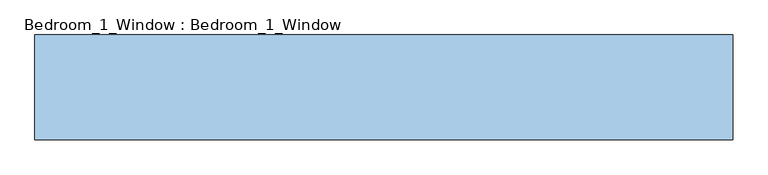
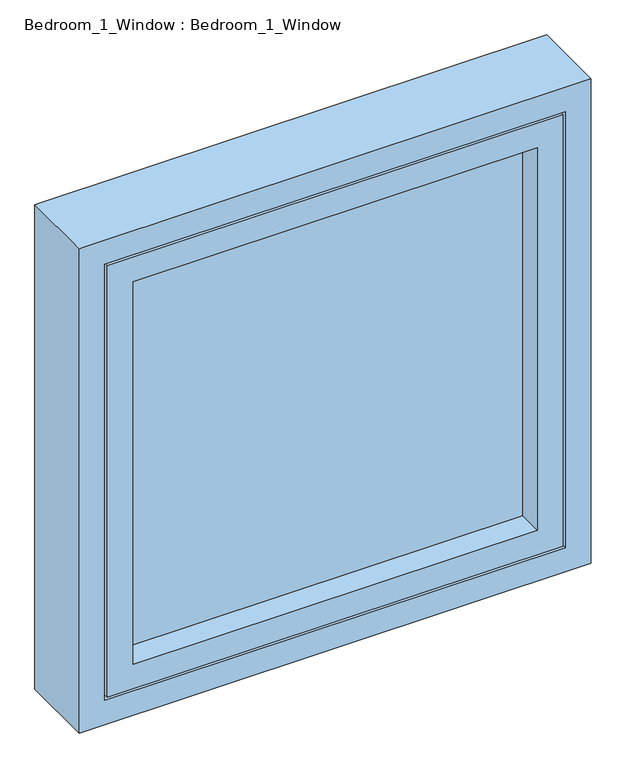
"""IFC4 building model written with IfcOpenShell, lengths in millimetres: window geometry, Bedroom_1_Window : Bedroom_1_Window."""

import ifcopenshell
import ifcopenshell.guid

model = None  # the IFC model being written
_history = None  # IfcOwnerHistory: only IFC2X3 demands one
_inside = {}  # id of a spatial element -> (the spatial element, [elements in it])
_under = {}  # id of a project, library or spatial element -> (it, [spatial elements below it])
_declared = {}  # id of a project -> (the project, [libraries it declares])
_typed = {}  # id of a type object -> (the type object, [elements of that type])
_made_of = {}  # id of a material, layer set ... -> (it, [elements and type objects made of it])


def new_model(schema):
    """Start an empty IFC model of exactly this schema.

    Asked for "IFC4X3", IfcOpenShell would pick the latest addendum, in which some entities
    have other attributes; the version numbers below select the first issue.
    IFC2X3 requires an IfcOwnerHistory on every rooted entity: one is made here for all.
    """
    global model, _history
    if schema == "IFC4X3":
        model = ifcopenshell.file(schema_version=(4, 3, 0, 0))
    else:
        model = ifcopenshell.file(schema=schema)
    _inside.clear()
    _under.clear()
    _declared.clear()
    _typed.clear()
    _made_of.clear()
    _history = None
    if model.schema == "IFC2X3":
        org = make("IfcOrganization", Name="unknown")
        user = make(
            "IfcPersonAndOrganization",
            ThePerson=make("IfcPerson", FamilyName="unknown"),
            TheOrganization=org,
        )
        app = make(
            "IfcApplication",
            ApplicationDeveloper=org,
            Version="unknown",
            ApplicationFullName="unknown",
            ApplicationIdentifier="unknown",
        )
        _history = make(
            "IfcOwnerHistory",
            OwningUser=user,
            OwningApplication=app,
            ChangeAction="ADDED",
            CreationDate=0,
        )
    return model


def make(cls, **values):
    """One entity of the class cls with the attributes given. An attribute that is None is left unset."""
    return model.create_entity(
        cls, **{name: value for name, value in values.items() if value is not None}
    )


def rooted(cls, **values):
    """An entity with a GlobalId (a new one), such as an element, a storey or a relation."""
    return make(cls, GlobalId=ifcopenshell.guid.new(), OwnerHistory=_history, **values)


def si_unit(unit_type, name, prefix=None):
    """IfcSIUnit, for example si_unit("LENGTHUNIT", "METRE", prefix="MILLI")."""
    return make("IfcSIUnit", UnitType=unit_type, Prefix=prefix, Name=name)


def assignment(units):
    """IfcUnitAssignment: the units of a project."""
    return None if units is None else make("IfcUnitAssignment", Units=units)


def point(xyz):
    """IfcCartesianPoint."""
    return None if xyz is None else make("IfcCartesianPoint", Coordinates=xyz)


def direction(xyz):
    """IfcDirection."""
    return None if xyz is None else make("IfcDirection", DirectionRatios=xyz)


def frame(location, z_axis=None, x_axis=None):
    """IfcAxis2Placement3D, a coordinate frame: its origin and axes. An axis left out is left unset."""
    return make(
        "IfcAxis2Placement3D",
        Location=point(location),
        Axis=direction(z_axis),
        RefDirection=direction(x_axis),
    )


def origin():
    """The frame at (0, 0, 0) with its axes left unset."""
    return frame((0.0, 0.0, 0.0))


def place(relative_to, where):
    """IfcLocalPlacement: puts the frame where relative to a parent placement (None: the world)."""
    return make(
        "IfcLocalPlacement", PlacementRelTo=relative_to, RelativePlacement=where
    )


def context(
    kind, dimensions, precision=None, world=None, true_north=None, identifier=None
):
    """IfcGeometricRepresentationContext, for example the 3D "Model" context."""
    return make(
        "IfcGeometricRepresentationContext",
        ContextIdentifier=identifier,
        ContextType=kind,
        CoordinateSpaceDimension=dimensions,
        Precision=precision,
        WorldCoordinateSystem=world,
        TrueNorth=true_north,
    )


def project(units=None, contexts=None):
    """IfcProject with its units and contexts."""
    return rooted(
        "IfcProject",
        Name="project",
        RepresentationContexts=contexts,
        UnitsInContext=assignment(units),
    )


def spatial(cls, under=None, at=None, **own):
    """A site, building, storey or space (cls), placed at a placement, below another one or the project."""
    s = rooted(cls, ObjectPlacement=at, **own)
    if under is not None:
        _under.setdefault(under.id(), (under, []))[1].append(s)
    return s


def polyline(points):
    """IfcPolyline through the points."""
    return make("IfcPolyline", Points=[point(p) for p in points])


def outline(outer, holes=None, kind="AREA"):
    """IfcArbitraryClosedProfileDef: a profile drawn as a closed curve; with holes, ...WithVoids."""
    if holes is None:
        return make("IfcArbitraryClosedProfileDef", ProfileType=kind, OuterCurve=outer)
    return make(
        "IfcArbitraryProfileDefWithVoids",
        ProfileType=kind,
        OuterCurve=outer,
        InnerCurves=holes,
    )


def extrude(swept, where, along, depth):
    """IfcExtrudedAreaSolid: the profile swept, set in the frame where, extruded along a direction by depth."""
    return make(
        "IfcExtrudedAreaSolid",
        SweptArea=swept,
        Position=where,
        ExtrudedDirection=direction(along),
        Depth=depth,
    )


def shape(context_of_items, identifier, shape_type, items):
    """IfcShapeRepresentation: the items that make up one representation, for example the "Body"."""
    return make(
        "IfcShapeRepresentation",
        ContextOfItems=context_of_items,
        RepresentationIdentifier=identifier,
        RepresentationType=shape_type,
        Items=items,
    )


def source(mapping_origin, context_of_items, identifier, shape_type, items):
    """IfcRepresentationMap: a shape defined once, which mapped items show again and again."""
    return make(
        "IfcRepresentationMap",
        MappingOrigin=mapping_origin,
        MappedRepresentation=shape(context_of_items, identifier, shape_type, items),
    )


def transform(
    local_origin,
    x_axis=None,
    y_axis=None,
    z_axis=None,
    scale=None,
    scale2=None,
    scale3=None,
    uniform=True,
):
    """IfcCartesianTransformationOperator3D, or its non-uniform kind. x_axis, y_axis, z_axis: its Axis1, 2, 3."""
    if uniform:
        return make(
            "IfcCartesianTransformationOperator3D",
            Axis1=direction(x_axis),
            Axis2=direction(y_axis),
            LocalOrigin=point(local_origin),
            Scale=scale,
            Axis3=direction(z_axis),
        )
    return make(
        "IfcCartesianTransformationOperator3DnonUniform",
        Axis1=direction(x_axis),
        Axis2=direction(y_axis),
        LocalOrigin=point(local_origin),
        Scale=scale,
        Axis3=direction(z_axis),
        Scale2=scale2,
        Scale3=scale3,
    )


def mapped(mapping_source, mapping_target):
    """IfcMappedItem: shows the shape of a source again, moved by a transform."""
    return make(
        "IfcMappedItem", MappingSource=mapping_source, MappingTarget=mapping_target
    )


def made_of(thing, what):
    """Note that an element or type object is made of a material, layer set ...; save() writes the relation."""
    if what is not None:
        _made_of.setdefault(what.id(), (what, []))[1].append(thing)
    return thing


def element(
    cls,
    number,
    at=None,
    inside=None,
    cuts=None,
    type_object=None,
    material=None,
    context=None,
    identifier="Body",
    shape_type=None,
    held_by="IfcProductDefinitionShape",
    body=None,
    shapes=None,
    **own,
):
    """One element of the class cls, such as IfcWall. Its Tag is "e" and its number.

    at: its placement. inside: the storey or other place that contains it. cuts: it is an
    opening in that element (IfcRelVoidsElement). A single representation is given by context,
    identifier, shape_type and body (its items); several are given by shapes. held_by: the class
    of the entity that holds the representations. save() writes the other relations.
    """
    e = rooted(cls, Tag="e%d" % number, ObjectPlacement=at, **own)
    if body is not None:
        shapes = [shape(context, identifier, shape_type, body)]
    if shapes is not None:
        e.Representation = make(held_by, Representations=shapes)
    if inside is not None:
        _inside.setdefault(inside.id(), (inside, []))[1].append(e)
    if cuts is not None:
        rooted(
            "IfcRelVoidsElement", RelatingBuildingElement=cuts, RelatedOpeningElement=e
        )
    if type_object is not None:
        _typed.setdefault(type_object.id(), (type_object, []))[1].append(e)
    return made_of(e, material)


def aggregate(whole, parts):
    """IfcRelAggregates: a whole, such as a stair, and the parts it consists of."""
    return rooted("IfcRelAggregates", RelatingObject=whole, RelatedObjects=parts)


def save(model, path):
    """Write the relations noted so far, then the file.

    IfcRelAggregates (storeys below a building ...), IfcRelContainedInSpatialStructure (elements
    in a storey), IfcRelDefinesByType, IfcRelAssociatesMaterial and IfcRelDeclares: one each for
    every whole, place, type object, material and project.
    """
    for whole, parts in _under.values():
        aggregate(whole, parts)
    for where, things in _inside.values():
        rooted(
            "IfcRelContainedInSpatialStructure",
            RelatedElements=things,
            RelatingStructure=where,
        )
    for kind, things in _typed.values():
        rooted("IfcRelDefinesByType", RelatedObjects=things, RelatingType=kind)
    for what, things in _made_of.values():
        rooted("IfcRelAssociatesMaterial", RelatedObjects=things, RelatingMaterial=what)
    for by, libraries in _declared.values():
        rooted("IfcRelDeclares", RelatingContext=by, RelatedDefinitions=libraries)
    model.write(path)


def bedroom_1_window_bedroom_1_window_a7b937d5(model_context):
    return source(origin(), model_context, "Body", "SweptSolid", [
        extrude(outline(polyline([(5180.0, 12115.0), (5970.0, 12115.0), (5970.0, 12105.0), (5180.0, 12105.0), (5180.0, 12115.0)])), frame((0.0, 0.0, 1555.0), z_axis=(0.0, 0.0, 1.0), x_axis=(1.0, 0.0, 0.0)), (0.0, 0.0, 1.0), 790.0),
        extrude(outline(polyline([(1505.0, 6020.0), (2395.0, 6020.0), (2395.0, 5130.0), (1505.0, 5130.0), (1505.0, 6020.0)]), holes=[polyline([(1555.0, 5180.0), (2345.0, 5180.0), (2345.0, 5970.0), (1555.0, 5970.0), (1555.0, 5180.0)])]), frame((0.0, 12055.0, 0.0), z_axis=(0.0, 1.0, 0.0), x_axis=(0.0, 0.0, 1.0)), (0.0, 0.0, 1.0), 100.0),
        extrude(outline(polyline([(1450.0, 6075.0), (2450.0, 6075.0), (2450.0, 5075.0), (1450.0, 5075.0), (1450.0, 6075.0)]), holes=[polyline([(1500.0, 5125.0), (2400.0, 5125.0), (2400.0, 6025.0), (1500.0, 6025.0), (1500.0, 5125.0)])]), frame((0.0, 12055.0, 0.0), z_axis=(0.0, 1.0, 0.0), x_axis=(0.0, 0.0, 1.0)), (0.0, 0.0, 1.0), 150.0),
    ])


if __name__ == "__main__":
    model = new_model("IFC4")
    model_context = context("Model", 3, world=origin())
    ifc_project = project(units=[si_unit("LENGTHUNIT", "METRE", prefix="MILLI")], contexts=[model_context])
    site = spatial("IfcSite", under=ifc_project)
    building = spatial("IfcBuilding", under=site)
    placement = place(None, origin())
    bedroom_1_window_bedroom_1_window_shape = bedroom_1_window_bedroom_1_window_a7b937d5(model_context)
    element("IfcWindow", 1, ObjectType="Bedroom_1_Window : Bedroom_1_Window", at=placement, inside=building, context=model_context, shape_type="MappedRepresentation", body=[
        mapped(bedroom_1_window_bedroom_1_window_shape, transform((0.0, 0.0, 0.0), x_axis=(1.0, 0.0, 0.0), y_axis=(0.0, 1.0, 0.0), z_axis=(0.0, 0.0, 1.0))),
    ])
    save(model, "model.ifc")

# Revit data of these elements
# Type "Bedroom_1_Window : Bedroom_1_Window"
#   Type Mark = "52"
#   NameOverride = "Bedroom_1_Window"
# Element 1 (IfcWindow, "Bedroom_1_Window : Bedroom_1_Window")
#   Materials on its faces: "IfcSurfaceStyle #392", "IfcSurfaceStyle #398"
# Materials
#   "IfcSurfaceStyle #392": class "Unassigned", colour RGB 204 204 204, transparency 0
#   "IfcSurfaceStyle #398": class "Unassigned", colour RGB 93 183 203, transparency 0.85
